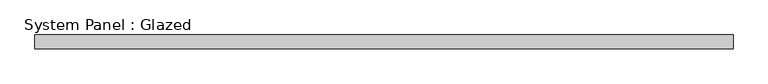
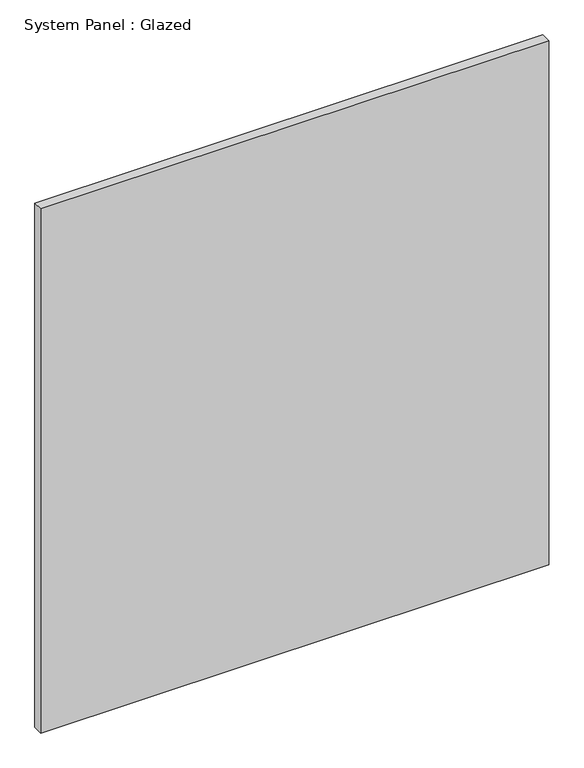
"""IFC4 building model written with IfcOpenShell, lengths in millimetres: plate geometry, System Panel : Glazed."""

from ifc_helpers import new_model, si_unit, origin, origin_with_axes, place, context, project, spatial, polyline, outline, extrude, source, transform, mapped, element, save


def system_panel_glazed_097b625c(model_context):
    return source(origin(), model_context, "Body", "SweptSolid", [
        extrude(outline(polyline([(641.6666667, 24.5), (-641.6666667, 24.5), (-641.6666667, 49.5), (641.6666667, 49.5), (641.6666667, 24.5)])), origin_with_axes(), (0.0, 0.0, 1.0), 1400.0),
    ])


if __name__ == "__main__":
    model = new_model("IFC4")
    model_context = context("Model", 3, world=origin())
    ifc_project = project(units=[si_unit("LENGTHUNIT", "METRE", prefix="MILLI")], contexts=[model_context])
    site = spatial("IfcSite", under=ifc_project)
    building = spatial("IfcBuilding", under=site)
    placement = place(None, origin())
    system_panel_glazed_shape = system_panel_glazed_097b625c(model_context)
    element("IfcPlate", 1, ObjectType="System Panel : Glazed", at=placement, inside=building, context=model_context, shape_type="MappedRepresentation", body=[
        mapped(system_panel_glazed_shape, transform((0.0, 0.0, 0.0), x_axis=(1.0, 0.0, 0.0), y_axis=(0.0, 1.0, 0.0), z_axis=(0.0, 0.0, 1.0))),
    ])
    save(model, "model.ifc")

# Revit data of these elements
# Element 1 (IfcPlate, "System Panel : Glazed")
#   Materials on its faces: "Glass"
# Materials
#   "Glass": class "Glass", colour RGB 0 128 192, transparency 0.9
